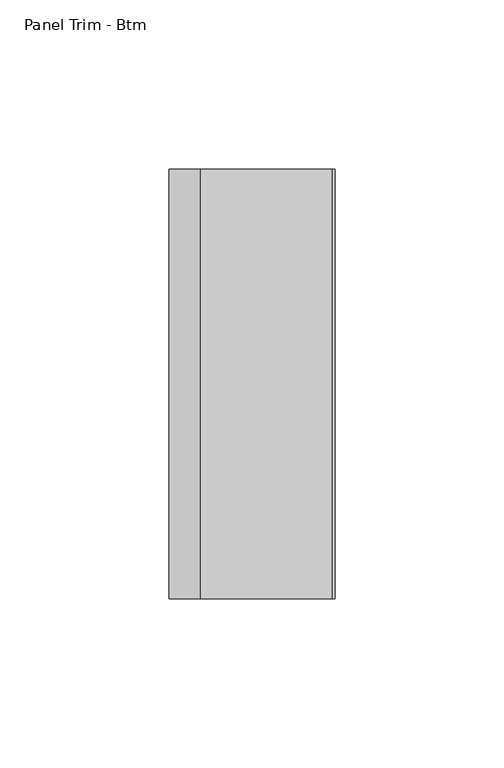
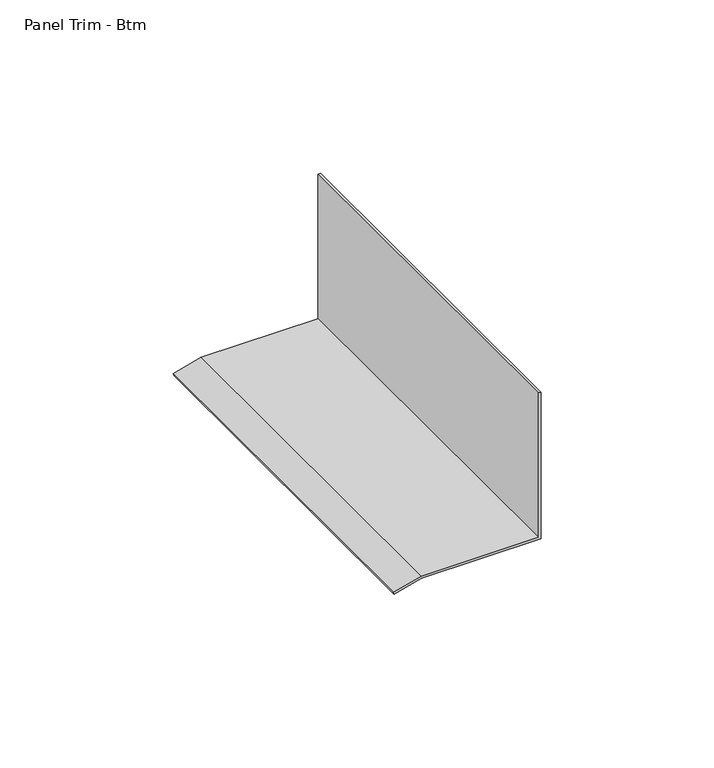
"""IFC4 building model written with IfcOpenShell, lengths in millimetres: proxy geometry, Btm Trim - Mull : Panel Trim - Btm."""

import ifcopenshell
import ifcopenshell.guid

model = None  # the IFC model being written
_history = None  # IfcOwnerHistory: only IFC2X3 demands one
_inside = {}  # id of a spatial element -> (the spatial element, [elements in it])
_under = {}  # id of a project, library or spatial element -> (it, [spatial elements below it])
_declared = {}  # id of a project -> (the project, [libraries it declares])
_typed = {}  # id of a type object -> (the type object, [elements of that type])
_made_of = {}  # id of a material, layer set ... -> (it, [elements and type objects made of it])


def new_model(schema):
    """Start an empty IFC model of exactly this schema.

    Asked for "IFC4X3", IfcOpenShell would pick the latest addendum, in which some entities
    have other attributes; the version numbers below select the first issue.
    IFC2X3 requires an IfcOwnerHistory on every rooted entity: one is made here for all.
    """
    global model, _history
    if schema == "IFC4X3":
        model = ifcopenshell.file(schema_version=(4, 3, 0, 0))
    else:
        model = ifcopenshell.file(schema=schema)
    _inside.clear()
    _under.clear()
    _declared.clear()
    _typed.clear()
    _made_of.clear()
    _history = None
    if model.schema == "IFC2X3":
        org = make("IfcOrganization", Name="unknown")
        user = make(
            "IfcPersonAndOrganization",
            ThePerson=make("IfcPerson", FamilyName="unknown"),
            TheOrganization=org,
        )
        app = make(
            "IfcApplication",
            ApplicationDeveloper=org,
            Version="unknown",
            ApplicationFullName="unknown",
            ApplicationIdentifier="unknown",
        )
        _history = make(
            "IfcOwnerHistory",
            OwningUser=user,
            OwningApplication=app,
            ChangeAction="ADDED",
            CreationDate=0,
        )
    return model


def make(cls, **values):
    """One entity of the class cls with the attributes given. An attribute that is None is left unset."""
    return model.create_entity(
        cls, **{name: value for name, value in values.items() if value is not None}
    )


def rooted(cls, **values):
    """An entity with a GlobalId (a new one), such as an element, a storey or a relation."""
    return make(cls, GlobalId=ifcopenshell.guid.new(), OwnerHistory=_history, **values)


def si_unit(unit_type, name, prefix=None):
    """IfcSIUnit, for example si_unit("LENGTHUNIT", "METRE", prefix="MILLI")."""
    return make("IfcSIUnit", UnitType=unit_type, Prefix=prefix, Name=name)


def assignment(units):
    """IfcUnitAssignment: the units of a project."""
    return None if units is None else make("IfcUnitAssignment", Units=units)


def point(xyz):
    """IfcCartesianPoint."""
    return None if xyz is None else make("IfcCartesianPoint", Coordinates=xyz)


def direction(xyz):
    """IfcDirection."""
    return None if xyz is None else make("IfcDirection", DirectionRatios=xyz)


def frame(location, z_axis=None, x_axis=None):
    """IfcAxis2Placement3D, a coordinate frame: its origin and axes. An axis left out is left unset."""
    return make(
        "IfcAxis2Placement3D",
        Location=point(location),
        Axis=direction(z_axis),
        RefDirection=direction(x_axis),
    )


def origin():
    """The frame at (0, 0, 0) with its axes left unset."""
    return frame((0.0, 0.0, 0.0))


def place(relative_to, where):
    """IfcLocalPlacement: puts the frame where relative to a parent placement (None: the world)."""
    return make(
        "IfcLocalPlacement", PlacementRelTo=relative_to, RelativePlacement=where
    )


def context(
    kind, dimensions, precision=None, world=None, true_north=None, identifier=None
):
    """IfcGeometricRepresentationContext, for example the 3D "Model" context."""
    return make(
        "IfcGeometricRepresentationContext",
        ContextIdentifier=identifier,
        ContextType=kind,
        CoordinateSpaceDimension=dimensions,
        Precision=precision,
        WorldCoordinateSystem=world,
        TrueNorth=true_north,
    )


def project(units=None, contexts=None):
    """IfcProject with its units and contexts."""
    return rooted(
        "IfcProject",
        Name="project",
        RepresentationContexts=contexts,
        UnitsInContext=assignment(units),
    )


def spatial(cls, under=None, at=None, **own):
    """A site, building, storey or space (cls), placed at a placement, below another one or the project."""
    s = rooted(cls, ObjectPlacement=at, **own)
    if under is not None:
        _under.setdefault(under.id(), (under, []))[1].append(s)
    return s


def polyline(points):
    """IfcPolyline through the points."""
    return make("IfcPolyline", Points=[point(p) for p in points])


def outline(outer, holes=None, kind="AREA"):
    """IfcArbitraryClosedProfileDef: a profile drawn as a closed curve; with holes, ...WithVoids."""
    if holes is None:
        return make("IfcArbitraryClosedProfileDef", ProfileType=kind, OuterCurve=outer)
    return make(
        "IfcArbitraryProfileDefWithVoids",
        ProfileType=kind,
        OuterCurve=outer,
        InnerCurves=holes,
    )


def extrude(swept, where, along, depth):
    """IfcExtrudedAreaSolid: the profile swept, set in the frame where, extruded along a direction by depth."""
    return make(
        "IfcExtrudedAreaSolid",
        SweptArea=swept,
        Position=where,
        ExtrudedDirection=direction(along),
        Depth=depth,
    )


def shape(context_of_items, identifier, shape_type, items):
    """IfcShapeRepresentation: the items that make up one representation, for example the "Body"."""
    return make(
        "IfcShapeRepresentation",
        ContextOfItems=context_of_items,
        RepresentationIdentifier=identifier,
        RepresentationType=shape_type,
        Items=items,
    )


def source(mapping_origin, context_of_items, identifier, shape_type, items):
    """IfcRepresentationMap: a shape defined once, which mapped items show again and again."""
    return make(
        "IfcRepresentationMap",
        MappingOrigin=mapping_origin,
        MappedRepresentation=shape(context_of_items, identifier, shape_type, items),
    )


def transform(
    local_origin,
    x_axis=None,
    y_axis=None,
    z_axis=None,
    scale=None,
    scale2=None,
    scale3=None,
    uniform=True,
):
    """IfcCartesianTransformationOperator3D, or its non-uniform kind. x_axis, y_axis, z_axis: its Axis1, 2, 3."""
    if uniform:
        return make(
            "IfcCartesianTransformationOperator3D",
            Axis1=direction(x_axis),
            Axis2=direction(y_axis),
            LocalOrigin=point(local_origin),
            Scale=scale,
            Axis3=direction(z_axis),
        )
    return make(
        "IfcCartesianTransformationOperator3DnonUniform",
        Axis1=direction(x_axis),
        Axis2=direction(y_axis),
        LocalOrigin=point(local_origin),
        Scale=scale,
        Axis3=direction(z_axis),
        Scale2=scale2,
        Scale3=scale3,
    )


def mapped(mapping_source, mapping_target):
    """IfcMappedItem: shows the shape of a source again, moved by a transform."""
    return make(
        "IfcMappedItem", MappingSource=mapping_source, MappingTarget=mapping_target
    )


def made_of(thing, what):
    """Note that an element or type object is made of a material, layer set ...; save() writes the relation."""
    if what is not None:
        _made_of.setdefault(what.id(), (what, []))[1].append(thing)
    return thing


def element(
    cls,
    number,
    at=None,
    inside=None,
    cuts=None,
    type_object=None,
    material=None,
    context=None,
    identifier="Body",
    shape_type=None,
    held_by="IfcProductDefinitionShape",
    body=None,
    shapes=None,
    **own,
):
    """One element of the class cls, such as IfcWall. Its Tag is "e" and its number.

    at: its placement. inside: the storey or other place that contains it. cuts: it is an
    opening in that element (IfcRelVoidsElement). A single representation is given by context,
    identifier, shape_type and body (its items); several are given by shapes. held_by: the class
    of the entity that holds the representations. save() writes the other relations.
    """
    e = rooted(cls, Tag="e%d" % number, ObjectPlacement=at, **own)
    if body is not None:
        shapes = [shape(context, identifier, shape_type, body)]
    if shapes is not None:
        e.Representation = make(held_by, Representations=shapes)
    if inside is not None:
        _inside.setdefault(inside.id(), (inside, []))[1].append(e)
    if cuts is not None:
        rooted(
            "IfcRelVoidsElement", RelatingBuildingElement=cuts, RelatedOpeningElement=e
        )
    if type_object is not None:
        _typed.setdefault(type_object.id(), (type_object, []))[1].append(e)
    return made_of(e, material)


def aggregate(whole, parts):
    """IfcRelAggregates: a whole, such as a stair, and the parts it consists of."""
    return rooted("IfcRelAggregates", RelatingObject=whole, RelatedObjects=parts)


def save(model, path):
    """Write the relations noted so far, then the file.

    IfcRelAggregates (storeys below a building ...), IfcRelContainedInSpatialStructure (elements
    in a storey), IfcRelDefinesByType, IfcRelAssociatesMaterial and IfcRelDeclares: one each for
    every whole, place, type object, material and project.
    """
    for whole, parts in _under.values():
        aggregate(whole, parts)
    for where, things in _inside.values():
        rooted(
            "IfcRelContainedInSpatialStructure",
            RelatedElements=things,
            RelatingStructure=where,
        )
    for kind, things in _typed.values():
        rooted("IfcRelDefinesByType", RelatedObjects=things, RelatingType=kind)
    for what, things in _made_of.values():
        rooted("IfcRelAssociatesMaterial", RelatedObjects=things, RelatingMaterial=what)
    for by, libraries in _declared.values():
        rooted("IfcRelDeclares", RelatingContext=by, RelatedDefinitions=libraries)
    model.write(path)


def panel_trim_btm_a4ea7572(model_context):
    return source(origin(), model_context, "Body", "SweptSolid", [
        extrude(outline(polyline([(12.7, 587326.1141748), (10.2077022, 587316.8127928), (9.4409986, 587317.0182304), (11.90625, 587326.2186739), (11.90625, 587365.8934739), (63.5, 587365.8934739), (63.5, 587365.1060739), (12.7, 587365.1060739), (12.7, 587326.1141748)])), frame((0.0, -536420.7663841, 0.0), z_axis=(0.0, 1.0, 0.0), x_axis=(0.0, 0.0, 1.0)), (0.0, 0.0, 1.0), 127.0),
    ])


if __name__ == "__main__":
    model = new_model("IFC4")
    model_context = context("Model", 3, world=origin())
    ifc_project = project(units=[si_unit("LENGTHUNIT", "METRE", prefix="MILLI")], contexts=[model_context])
    site = spatial("IfcSite", under=ifc_project)
    building = spatial("IfcBuilding", under=site)
    placement = place(None, origin())
    panel_trim_btm_shape = panel_trim_btm_a4ea7572(model_context)
    element("IfcBuildingElementProxy", 1, Name="Btm Trim - Mull : Panel Trim - Btm", ObjectType="Btm Trim - Mull : Panel Trim - Btm", at=placement, inside=building, context=model_context, shape_type="MappedRepresentation", body=[
        mapped(panel_trim_btm_shape, transform((0.0, 0.0, 0.0), x_axis=(1.0, 0.0, 0.0), y_axis=(0.0, 1.0, 0.0), z_axis=(0.0, 0.0, 1.0))),
    ])
    save(model, "model.ifc")

# Revit data of these elements
# Element 1 (IfcBuildingElementProxy, "Btm Trim - Mull : Panel Trim - Btm")
#   Materials on its faces: "BASE TRIM BY MTL PANEL MFR."
# Materials
#   "BASE TRIM BY MTL PANEL MFR.": class "Generic", colour RGB 239 242 240, transparency 0, Cost = 0
